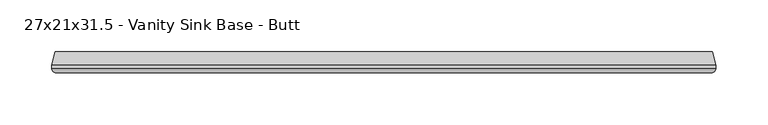
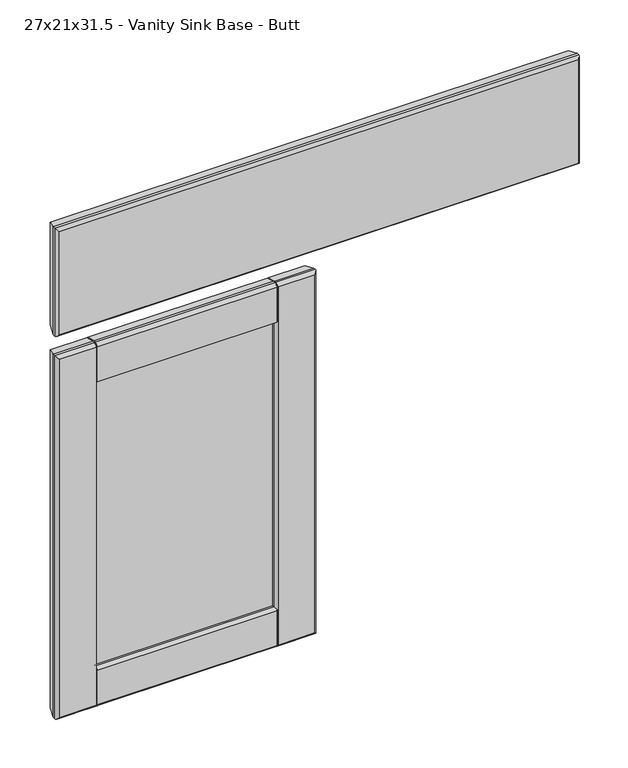
"""IFC4 building model written with IfcOpenShell, lengths in millimetres: furniture geometry, Cabinet-Base-Merillat-Double_Door-Marlin : 27x21x31.5 - Vanity Sink Base - Butt."""

from ifc_helpers import new_model, si_unit, frame, origin, place, context, project, spatial, polyline, circle_curve, ellipse_curve, outline, extrude, source, transform, mapped, element, save
from ifc_brep_helpers import plane_surface, cylinder_surface, advanced_brep


def furniture_27x21x31_5_vanity_sink_base_butt_8131d798(model_context):
    return source(origin(), model_context, "Body", "SolidModel", [
        advanced_brep(
        [(-298.8408026, -629.92, 771.6035075), (-298.8408026, -629.92, 638.0964925), (336.3162124, -629.92, 638.0964925), (336.3162124, -629.92, 771.6035075), (-298.4320951, -609.6, 638.5052), (-298.4320951, -609.6, 771.1948), (335.9075049, -609.6, 771.1948), (335.9075049, -609.6, 638.5052), (-301.9372951, -625.4496, 774.7), (-301.9372951, -622.681, 774.7), (-301.9372951, -622.681, 635.0), (-301.9372951, -625.4496, 635.0), (339.4127049, -622.681, 635.0), (339.4127049, -625.4496, 635.0), (339.4127049, -622.681, 774.7), (339.4127049, -625.4496, 774.7)],
        [
            (0, 1),
            (1, 2),
            (2, 3),
            (3, 0),
            (4, 5),
            (5, 6),
            (6, 7),
            (7, 4),
            (8, 9),
            (9, 10),
            (10, 11),
            (11, 8),
            (10, 12),
            (12, 13),
            (13, 11),
            (12, 14),
            (14, 15),
            (15, 13),
            (8, 15),
            (14, 9),
            (11, 1, ellipse_curve(frame((-297.1620951, -625.4496, 639.7752), z_axis=(-0.7071067811865475, 0.0, 0.7071067811865475), x_axis=(-0.7071067811865474, 0.0, -0.7071067811865476)), 6.7531526, 4.7752)),
            (0, 8, ellipse_curve(frame((-297.1620951, -625.4496, 769.9248), z_axis=(-0.7071067811865475, 0.0, -0.7071067811865475), x_axis=(0.7071067811865474, 0.0, -0.7071067811865476)), 6.7531526, 4.7752)),
            (4, 10),
            (9, 5),
            (13, 2, ellipse_curve(frame((334.6375049, -625.4496, 639.7752), z_axis=(-0.7071067811865475, 0.0, -0.7071067811865475), x_axis=(0.7071067811865476, 0.0, -0.7071067811865474)), 6.7531526, 4.7752)),
            (7, 12),
            (15, 3, ellipse_curve(frame((334.6375049, -625.4496, 769.9248), z_axis=(0.7071067811865475, 0.0, -0.7071067811865475), x_axis=(0.7071067811865474, 0.0, 0.7071067811865476)), 6.7531526, 4.7752)),
            (6, 14),
        ],
        [
            plane_surface(frame((-301.9372951, -629.92, 774.7), z_axis=(0.0, -1.0, 0.0), x_axis=(0.0, 0.0, -1.0))),
            plane_surface(frame((-301.9372951, -609.6, 774.7), z_axis=(0.0, 1.0, 0.0), x_axis=(0.0, 0.0, 1.0))),
            plane_surface(frame((-301.9372951, -629.92, 774.7), z_axis=(-1.0, 0.0, 0.0), x_axis=(0.0, 1.0, 0.0))),
            plane_surface(frame((-301.9372951, -629.92, 635.0), z_axis=(0.0, 0.0, -1.0), x_axis=(0.0, 1.0, 0.0))),
            plane_surface(frame((339.4127049, -629.92, 635.0), z_axis=(1.0, 0.0, 0.0), x_axis=(0.0, 1.0, 0.0))),
            plane_surface(frame((339.4127049, -629.92, 774.7), z_axis=(0.0, 0.0, 1.0), x_axis=(0.0, 1.0, 0.0))),
            cylinder_surface(frame((-297.1620951, -625.4496, 774.7), z_axis=(0.0, 0.0, -1.0), x_axis=(0.0, 1.0, 0.0)), 4.7752),
            plane_surface(frame((-301.9372951, -622.681, 774.7), z_axis=(-0.9659229350723619, 0.25882983502910506, 0.0), x_axis=(0.0, 0.0, -1.0))),
            cylinder_surface(frame((-301.9372951, -625.4496, 639.7752), z_axis=(1.0, 0.0, 0.0), x_axis=(0.0, 1.0, 0.0)), 4.7752),
            plane_surface(frame((-301.9372951, -622.681, 635.0), z_axis=(0.0, 0.25882983502910506, -0.9659229350723619), x_axis=(1.0, 0.0, 0.0))),
            cylinder_surface(frame((334.6375049, -625.4496, 635.0), z_axis=(0.0, 0.0, 1.0), x_axis=(0.0, 1.0, 0.0)), 4.7752),
            plane_surface(frame((339.4127049, -622.681, 635.0), z_axis=(0.9659229350723619, 0.25882983502910506, 0.0), x_axis=(0.0, 0.0, 1.0))),
            cylinder_surface(frame((339.4127049, -625.4496, 769.9248), z_axis=(-1.0, 0.0, 0.0), x_axis=(0.0, 1.0, 0.0)), 4.7752),
            plane_surface(frame((339.4127049, -622.681, 774.7), z_axis=(0.0, 0.25882983502910506, 0.9659229350723619), x_axis=(-1.0, 0.0, 0.0))),
        ],
        [
            (0, [[1, 2, 3, 4]]),
            (1, [[5, 6, 7, 8]]),
            (2, [[9, 10, 11, 12]]),
            (3, [[-11, 13, 14, 15]]),
            (4, [[-14, 16, 17, 18]]),
            (5, [[-9, 19, -17, 20]]),
            (6, [[21, -1, 22, -12]]),
            (7, [[23, -10, 24, -5]]),
            (8, [[-21, -15, 25, -2]]),
            (9, [[-23, -8, 26, -13]]),
            (10, [[-25, -18, 27, -3]]),
            (11, [[-26, -7, 28, -16]]),
            (12, [[-22, -4, -27, -19]]),
            (13, [[-24, -20, -28, -6]]),
        ],
    ),
        advanced_brep(
        [(-301.9372951, -625.4496, 609.6), (-301.9372951, -625.4496, 139.7), (-298.8408026, -629.92, 142.7964925), (-298.8408026, -629.92, 606.5035075), (-301.9372951, -622.681, 609.6), (-301.9372951, -622.681, 139.7), (-298.4320951, -609.6, 606.0948), (-298.4320951, -609.6, 143.2052), (-253.7361323, -609.6, 561.3988372), (-253.3660006, -610.39375, 561.0287055), (-251.2848416, -614.85681, 558.9475465), (-251.2848416, -614.85681, 190.3524535), (-253.3660006, -610.39375, 188.2712945), (-253.7361323, -609.6, 187.9011628), (-252.684611, -617.0969093, 560.347316), (-252.684611, -617.0969093, 188.952684), (-267.0122951, -617.347, 574.675), (-267.0122951, -617.347, 174.625), (-267.0122951, -622.173, 574.675), (-267.0122951, -622.173, 174.625), (-252.684611, -622.4230907, 560.347316), (-252.684611, -622.4230907, 188.952684), (-251.2848416, -624.66319, 558.9475465), (-251.2848416, -624.66319, 190.3524535), (-253.3660006, -629.12625, 561.0287055), (-253.7332649, -629.9138508, 561.3959698), (-253.7361323, -629.92, 187.9011628), (-253.3660006, -629.12625, 188.2712945), (14.0537124, -629.92, 142.7964925), (-31.0140137, -629.92, 142.7964925), (-31.0140137, -625.4496, 139.7), (17.1502049, -625.4496, 139.7), (-253.7332649, -625.4496, 139.7), (-253.7332649, -629.92, 142.7964925), (-252.1457649, -625.4496, 139.7), (-32.6015137, -625.4496, 139.7), (-32.6015137, -629.92, 142.7964925), (-252.1457649, -629.92, 142.7964925), (-31.0140137, -622.681, 139.7), (17.1502049, -622.681, 139.7), (-253.7332649, -622.681, 139.7), (-252.1457649, -622.681, 139.7), (-32.6015137, -622.681, 139.7), (-31.0140137, -609.6, 143.2052), (13.6450049, -609.6, 143.2052), (-252.1457649, -609.6, 143.2052), (-32.6015137, -609.6, 143.2052), (-253.7332649, -609.6, 143.2052), (-33.5022486, -614.85681, 190.3524535), (-31.4210895, -610.39375, 188.2712945), (-32.6015137, -610.39375, 188.2712945), (-32.6015137, -609.6, 187.9011628), (-252.1457649, -609.6, 187.9011628), (-252.1457649, -610.39375, 188.2712945), (-32.1024791, -617.0969093, 188.952684), (-17.7747951, -617.347, 174.625), (-17.7747951, -622.173, 174.625), (-32.1024791, -622.4230907, 188.952684), (-33.5022486, -624.66319, 190.3524535), (-252.1457649, -629.12625, 188.2712945), (-252.1457649, -629.92, 187.9011628), (-32.6015137, -629.92, 187.9011628), (-32.6015137, -629.12625, 188.2712945), (-31.4210895, -629.12625, 188.2712945), (17.1502049, -625.4496, 609.6), (14.0537124, -629.92, 606.5035075), (17.1502049, -622.681, 609.6), (13.6450049, -609.6, 606.0948), (-31.0509578, -609.6, 187.9011628), (-33.5022486, -614.85681, 558.9475465), (-31.4210895, -610.39375, 561.0287055), (-31.0509578, -609.6, 561.3988372), (-32.1024791, -617.0969093, 560.347316), (-17.7747951, -617.347, 574.675), (-17.7747951, -622.173, 574.675), (-32.1024791, -622.4230907, 560.347316), (-33.5022486, -624.66319, 558.9475465), (-31.0509578, -629.92, 187.9011628), (-31.0509578, -629.92, 561.3988372), (-31.4210895, -629.12625, 561.0287055), (-253.7332649, -629.92, 606.5035075), (-253.7332649, -625.4496, 609.6), (-31.0140137, -625.4496, 609.6), (-31.0140137, -629.92, 606.5035075), (-32.6015137, -625.4496, 609.6), (-252.1457649, -625.4496, 609.6), (-252.1457649, -629.92, 606.5035075), (-32.6015137, -629.92, 606.5035075), (-253.7332649, -622.681, 609.6), (-31.0140137, -622.681, 609.6), (-32.6015137, -622.681, 609.6), (-252.1457649, -622.681, 609.6), (-253.7332649, -609.6, 606.0948), (-31.0140137, -609.6, 606.0948), (-32.6015137, -609.6, 606.0948), (-252.1457649, -609.6, 606.0948), (-32.6015137, -609.6, 561.3988372), (-252.1457649, -609.6, 561.3988372), (-252.1457649, -610.39375, 561.0287055), (-32.6015137, -610.39375, 561.0287055), (-32.6015137, -629.12625, 561.0287055), (-32.6015137, -629.92, 561.3988372), (-252.1457649, -629.92, 561.3988372), (-252.1457649, -629.12625, 561.0287055), (-32.6015137, -629.12625, 606.3526052), (-32.6015137, -625.4496, 608.80625), (-32.6015137, -622.7855037, 608.80625), (-32.6015137, -610.39375, 605.4857412), (-31.0140137, -610.39375, 561.0287055), (-31.0140137, -610.39375, 605.4857412), (-31.0140137, -622.7855037, 608.80625), (-31.0140137, -625.4496, 608.80625), (-31.0140137, -629.12625, 606.3526052), (-31.0140137, -629.12625, 561.0287055), (-253.7332649, -629.12625, 561.0287055), (-253.7332649, -629.12625, 606.3526052), (-253.7332649, -625.4496, 608.80625), (-253.7332649, -622.7855037, 608.80625), (-253.7332649, -610.39375, 605.4857412), (-253.7332649, -610.39375, 561.0287055), (-252.1457649, -610.39375, 605.4857412), (-252.1457649, -622.7855037, 608.80625), (-252.1457649, -625.4496, 608.80625), (-252.1457649, -629.12625, 606.3526052), (-253.7332649, -610.39375, 188.2712945), (-253.7332649, -610.39375, 143.8142588), (-253.7332649, -622.7855037, 140.49375), (-253.7332649, -625.4496, 140.49375), (-253.7332649, -629.12625, 142.9473948), (-253.7332649, -629.12625, 188.2712945), (-252.1457649, -629.12625, 142.9473948), (-252.1457649, -625.4496, 140.49375), (-252.1457649, -622.7855037, 140.49375), (-252.1457649, -610.39375, 143.8142588), (-32.6015137, -610.39375, 143.8142588), (-32.6015137, -622.7855037, 140.49375), (-32.6015137, -625.4496, 140.49375), (-32.6015137, -629.12625, 142.9473948), (-31.0140137, -629.12625, 188.2712945), (-31.0140137, -629.12625, 142.9473948), (-31.0140137, -625.4496, 140.49375), (-31.0140137, -622.7855037, 140.49375), (-31.0140137, -610.39375, 143.8142588), (-31.0140137, -610.39375, 188.2712945)],
        [
            (0, 1),
            (1, 2, ellipse_curve(frame((-297.1620951, -625.4496, 144.4752), z_axis=(-0.7071067811865475, 0.0, 0.7071067811865475), x_axis=(0.7071067811865474, 0.0, 0.7071067811865476)), 6.7531526, 4.7752)),
            (2, 3),
            (3, 0, ellipse_curve(frame((-297.1620951, -625.4496, 604.8248), z_axis=(-0.7071067811865475, 0.0, -0.7071067811865475), x_axis=(-0.7071067811865474, 0.0, 0.7071067811865476)), 6.7531526, 4.7752)),
            (0, 4),
            (4, 5),
            (5, 1),
            (4, 6),
            (6, 7),
            (7, 5),
            (8, 9),
            (9, 10),
            (10, 11),
            (11, 12),
            (12, 13),
            (13, 8),
            (10, 14, ellipse_curve(frame((-252.7120951, -615.5223492, 560.3748), z_axis=(-0.7071067811865475, 0.0, -0.7071067811865475), x_axis=(-0.7071067811865474, 0.0, 0.7071067811865476)), 2.2271035, 1.5748)),
            (14, 15),
            (15, 11, ellipse_curve(frame((-252.7120951, -615.5223492, 188.9252), z_axis=(-0.7071067811865475, 0.0, 0.7071067811865475), x_axis=(0.7071067811865474, 0.0, 0.7071067811865476)), 2.2271035, 1.5748)),
            (14, 16),
            (16, 17),
            (17, 15),
            (16, 18),
            (18, 19),
            (19, 17),
            (18, 20),
            (20, 21),
            (21, 19),
            (20, 22, ellipse_curve(frame((-252.7120951, -623.9976508, 560.3748), z_axis=(-0.7071067811865475, 0.0, -0.7071067811865475), x_axis=(-0.7071067811865474, 0.0, 0.7071067811865476)), 2.2271035, 1.5748)),
            (22, 23),
            (23, 21, ellipse_curve(frame((-252.7120951, -623.9976508, 188.9252), z_axis=(-0.7071067811865475, 0.0, 0.7071067811865475), x_axis=(0.7071067811865474, 0.0, 0.7071067811865476)), 2.2271035, 1.5748)),
            (22, 24),
            (24, 25),
            (25, 26),
            (26, 27),
            (27, 23),
            (28, 29),
            (29, 30, circle_curve(frame((-31.0140137, -625.4496, 144.4752), z_axis=(1.0, 0.0, 0.0), x_axis=(0.0, 1.0, 0.0)), 4.7752)),
            (30, 31),
            (31, 28, ellipse_curve(frame((12.3750049, -625.4496, 144.4752), z_axis=(-0.7071067811865475, 0.0, -0.7071067811865475), x_axis=(-0.7071067811865476, 0.0, 0.7071067811865474)), 6.7531526, 4.7752)),
            (1, 32),
            (32, 33, circle_curve(frame((-253.7332649, -625.4496, 144.4752), z_axis=(-1.0, 0.0, 0.0), x_axis=(0.0, 1.0, 0.0)), 4.7752)),
            (33, 2),
            (34, 35),
            (35, 36, circle_curve(frame((-32.6015137, -625.4496, 144.4752), z_axis=(-1.0, 0.0, 0.0), x_axis=(0.0, 1.0, 0.0)), 4.7752)),
            (36, 37),
            (37, 34, circle_curve(frame((-252.1457649, -625.4496, 144.4752), z_axis=(1.0, 0.0, 0.0), x_axis=(0.0, 1.0, 0.0)), 4.7752)),
            (30, 38),
            (38, 39),
            (39, 31),
            (5, 40),
            (40, 32),
            (41, 42),
            (42, 35),
            (34, 41),
            (38, 43),
            (43, 44),
            (44, 39),
            (45, 46),
            (46, 42),
            (41, 45),
            (7, 47),
            (47, 40),
            (48, 49),
            (49, 50),
            (50, 51),
            (51, 52),
            (52, 53),
            (53, 12),
            (11, 48),
            (15, 54),
            (54, 48, ellipse_curve(frame((-32.0749951, -615.5223492, 188.9252), z_axis=(-0.7071067811865475, 0.0, -0.7071067811865475), x_axis=(-0.7071067811865476, 0.0, 0.7071067811865474)), 2.2271035, 1.5748)),
            (17, 55),
            (55, 54),
            (19, 56),
            (56, 55),
            (21, 57),
            (57, 56),
            (23, 58),
            (58, 57, ellipse_curve(frame((-32.0749951, -623.9976508, 188.9252), z_axis=(-0.7071067811865475, 0.0, -0.7071067811865475), x_axis=(-0.7071067811865476, 0.0, 0.7071067811865474)), 2.2271035, 1.5748)),
            (27, 59),
            (59, 60),
            (60, 61),
            (61, 62),
            (62, 63),
            (63, 58),
            (31, 64),
            (64, 65, ellipse_curve(frame((12.3750049, -625.4496, 604.8248), z_axis=(0.7071067811865475, 0.0, -0.7071067811865475), x_axis=(-0.7071067811865474, 0.0, -0.7071067811865476)), 6.7531526, 4.7752)),
            (65, 28),
            (39, 66),
            (66, 64),
            (44, 67),
            (67, 66),
            (68, 49),
            (48, 69),
            (69, 70),
            (70, 71),
            (71, 68),
            (54, 72),
            (72, 69, ellipse_curve(frame((-32.0749951, -615.5223492, 560.3748), z_axis=(0.7071067811865475, 0.0, -0.7071067811865475), x_axis=(-0.7071067811865474, 0.0, -0.7071067811865476)), 2.2271035, 1.5748)),
            (55, 73),
            (73, 72),
            (56, 74),
            (74, 73),
            (57, 75),
            (75, 74),
            (58, 76),
            (76, 75, ellipse_curve(frame((-32.0749951, -623.9976508, 560.3748), z_axis=(0.7071067811865475, 0.0, -0.7071067811865475), x_axis=(-0.7071067811865474, 0.0, -0.7071067811865476)), 2.2271035, 1.5748)),
            (63, 77),
            (77, 78),
            (78, 79),
            (79, 76),
            (3, 80),
            (80, 81, circle_curve(frame((-253.7332649, -625.4496, 604.8248), z_axis=(-1.0, 0.0, 0.0), x_axis=(0.0, 1.0, 0.0)), 4.7752)),
            (81, 0),
            (64, 82),
            (82, 83, circle_curve(frame((-31.0140137, -625.4496, 604.8248), z_axis=(1.0, 0.0, 0.0), x_axis=(0.0, 1.0, 0.0)), 4.7752)),
            (83, 65),
            (84, 85),
            (85, 86, circle_curve(frame((-252.1457649, -625.4496, 604.8248), z_axis=(1.0, 0.0, 0.0), x_axis=(0.0, 1.0, 0.0)), 4.7752)),
            (86, 87),
            (87, 84, circle_curve(frame((-32.6015137, -625.4496, 604.8248), z_axis=(-1.0, 0.0, 0.0), x_axis=(0.0, 1.0, 0.0)), 4.7752)),
            (81, 88),
            (88, 4),
            (66, 89),
            (89, 82),
            (90, 91),
            (91, 85),
            (84, 90),
            (88, 92),
            (92, 6),
            (67, 93),
            (93, 89),
            (94, 95),
            (95, 91),
            (90, 94),
            (51, 46),
            (45, 52),
            (43, 68),
            (71, 93),
            (92, 8),
            (13, 47),
            (96, 97),
            (97, 95),
            (94, 96),
            (9, 98),
            (98, 97),
            (96, 99),
            (99, 70),
            (69, 10),
            (72, 14),
            (73, 16),
            (74, 18),
            (75, 20),
            (76, 22),
            (79, 100),
            (100, 101),
            (101, 102),
            (102, 103),
            (103, 24),
            (33, 26),
            (25, 80),
            (36, 61),
            (60, 37),
            (83, 78),
            (77, 29),
            (86, 102),
            (101, 87),
            (100, 104),
            (104, 105, circle_curve(frame((-32.6015137, -625.4496, 604.8248), z_axis=(-1.0, 0.0, 0.0), x_axis=(0.0, 0.0, 1.0)), 3.98145)),
            (105, 106),
            (106, 107),
            (107, 99),
            (71, 108),
            (108, 109),
            (109, 110),
            (110, 111),
            (111, 112, circle_curve(frame((-31.0140137, -625.4496, 604.8248), z_axis=(1.0, 0.0, 0.0), x_axis=(0.0, 0.0, 1.0)), 3.98145)),
            (112, 113),
            (113, 78),
            (113, 79),
            (112, 104),
            (111, 105),
            (110, 106),
            (109, 107),
            (108, 70),
            (25, 114),
            (114, 115),
            (115, 116, circle_curve(frame((-253.7332649, -625.4496, 604.8248), z_axis=(-1.0, 0.0, 0.0), x_axis=(0.0, 0.0, 1.0)), 3.98145)),
            (116, 117),
            (117, 118),
            (118, 119),
            (119, 8),
            (98, 120),
            (120, 121),
            (121, 122),
            (122, 123, circle_curve(frame((-252.1457649, -625.4496, 604.8248), z_axis=(1.0, 0.0, 0.0), x_axis=(0.0, 0.0, 1.0)), 3.98145)),
            (123, 103),
            (24, 114),
            (123, 115),
            (122, 116),
            (121, 117),
            (120, 118),
            (9, 119),
            (13, 124),
            (124, 125),
            (125, 126),
            (126, 127),
            (127, 128, circle_curve(frame((-253.7332649, -625.4496, 144.4752), z_axis=(-1.0, 0.0, 0.0), x_axis=(0.0, 0.0, 1.0)), 3.98145)),
            (128, 129),
            (129, 26),
            (59, 130),
            (130, 131, circle_curve(frame((-252.1457649, -625.4496, 144.4752), z_axis=(1.0, 0.0, 0.0), x_axis=(0.0, 0.0, 1.0)), 3.98145)),
            (131, 132),
            (132, 133),
            (133, 53),
            (12, 124),
            (133, 125),
            (132, 126),
            (131, 127),
            (130, 128),
            (27, 129),
            (50, 134),
            (134, 135),
            (135, 136),
            (136, 137, circle_curve(frame((-32.6015137, -625.4496, 144.4752), z_axis=(-1.0, 0.0, 0.0), x_axis=(0.0, 0.0, 1.0)), 3.98145)),
            (137, 62),
            (138, 139),
            (139, 140, circle_curve(frame((-31.0140137, -625.4496, 144.4752), z_axis=(1.0, 0.0, 0.0), x_axis=(0.0, 0.0, 1.0)), 3.98145)),
            (140, 141),
            (141, 142),
            (142, 143),
            (143, 68),
            (77, 138),
            (63, 138),
            (143, 49),
            (142, 134),
            (141, 135),
            (140, 136),
            (139, 137),
        ],
        [
            cylinder_surface(frame((-297.1620951, -625.4496, 609.6), z_axis=(0.0, 0.0, 1.0), x_axis=(0.0, 1.0, 0.0)), 4.7752),
            plane_surface(frame((-301.9372951, -625.4496, 609.6), z_axis=(-1.0, 0.0, 0.0), x_axis=(0.0, 0.0, -1.0))),
            plane_surface(frame((-301.9372951, -622.681, 609.6), z_axis=(-0.9659229350723619, 0.25882983502910506, 0.0), x_axis=(0.0, 0.0, -1.0))),
            plane_surface(frame((-253.7361323, -609.6, 561.3988372), z_axis=(0.9063077870366099, 0.4226182617407856, 0.0), x_axis=(0.0, 0.0, -1.0))),
            cylinder_surface(frame((-252.7120951, -615.5223492, 609.6), z_axis=(0.0, 0.0, 1.0000000000000002), x_axis=(0.01745240643729364, -0.9998476951563912, 0.0)), 1.5748),
            plane_surface(frame((-252.684611, -617.0969093, 560.347316), z_axis=(0.017452406437322144, -0.9998476951563906, 0.0), x_axis=(0.0, 0.0, -1.0))),
            plane_surface(frame((-267.0122951, -617.347, 574.675), z_axis=(1.0, 0.0, 0.0), x_axis=(0.0, 0.0, -1.0))),
            plane_surface(frame((-267.0122951, -622.173, 574.675), z_axis=(0.01745240643727848, 0.9998476951563914, 0.0), x_axis=(0.0, 0.0, -1.0))),
            cylinder_surface(frame((-252.7120951, -623.9976508, 609.6), z_axis=(0.0, 0.0, 1.0000000000000002), x_axis=(0.9063077870367326, -0.42261826174052236, 0.0)), 1.5748),
            plane_surface(frame((-251.2848416, -624.66319, 558.9475465), z_axis=(0.9063077870366333, -0.4226182617407352, 0.0), x_axis=(0.0, 0.0, -1.0))),
            cylinder_surface(frame((-301.9372951, -625.4496, 144.4752), z_axis=(-1.0, 0.0, 0.0), x_axis=(0.0, 1.0, 0.0)), 4.7752),
            plane_surface(frame((-301.9372951, -625.4496, 139.7), z_axis=(0.0, 0.0, -1.0), x_axis=(1.0, 0.0, 0.0))),
            plane_surface(frame((-301.9372951, -622.681, 139.7), z_axis=(0.0, 0.25882983502910506, -0.9659229350723619), x_axis=(1.0, 0.0, 0.0))),
            plane_surface(frame((-253.7361323, -609.6, 187.9011628), z_axis=(0.0, 0.4226182617407856, 0.9063077870366099), x_axis=(1.0, 0.0, 0.0))),
            cylinder_surface(frame((-301.9372951, -615.5223492, 188.9252), z_axis=(-1.0000000000000002, 0.0, 0.0), x_axis=(0.0, -0.9998476951563912, 0.01745240643729364)), 1.5748),
            plane_surface(frame((-252.684611, -617.0969093, 188.952684), z_axis=(0.0, -0.9998476951563906, 0.017452406437322144), x_axis=(1.0, 0.0, 0.0))),
            plane_surface(frame((-267.0122951, -617.347, 174.625), z_axis=(0.0, 0.0, 1.0), x_axis=(1.0, 0.0, 0.0))),
            plane_surface(frame((-267.0122951, -622.173, 174.625), z_axis=(0.0, 0.9998476951563914, 0.01745240643727848), x_axis=(1.0, 0.0, 0.0))),
            cylinder_surface(frame((-301.9372951, -623.9976508, 188.9252), z_axis=(-1.0000000000000002, 0.0, 0.0), x_axis=(0.0, -0.42261826174052236, 0.9063077870367326)), 1.5748),
            plane_surface(frame((-251.2848416, -624.66319, 190.3524535), z_axis=(0.0, -0.4226182617407352, 0.9063077870366333), x_axis=(1.0, 0.0, 0.0))),
            cylinder_surface(frame((12.3750049, -625.4496, 139.7), z_axis=(0.0, 0.0, -1.0), x_axis=(0.0, 1.0, 0.0)), 4.7752),
            plane_surface(frame((17.1502049, -625.4496, 139.7), z_axis=(1.0, 0.0, 0.0), x_axis=(0.0, 0.0, 1.0))),
            plane_surface(frame((17.1502049, -622.681, 139.7), z_axis=(0.9659229350723619, 0.25882983502910506, 0.0), x_axis=(0.0, 0.0, 1.0))),
            plane_surface(frame((-31.0509578, -609.6, 187.9011628), z_axis=(-0.9063077870366099, 0.4226182617407856, 0.0), x_axis=(0.0, 0.0, 1.0))),
            cylinder_surface(frame((-32.0749951, -615.5223492, 139.7), z_axis=(0.0, 0.0, -1.0000000000000002), x_axis=(-0.01745240643729364, -0.9998476951563912, 0.0)), 1.5748),
            plane_surface(frame((-32.1024791, -617.0969093, 188.952684), z_axis=(-0.017452406437322144, -0.9998476951563906, 0.0), x_axis=(0.0, 0.0, 1.0))),
            plane_surface(frame((-17.7747951, -617.347, 174.625), z_axis=(-1.0, 0.0, 0.0), x_axis=(0.0, 0.0, 1.0))),
            plane_surface(frame((-17.7747951, -622.173, 174.625), z_axis=(-0.01745240643727848, 0.9998476951563914, 0.0), x_axis=(0.0, 0.0, 1.0))),
            cylinder_surface(frame((-32.0749951, -623.9976508, 139.7), z_axis=(0.0, 0.0, -1.0000000000000002), x_axis=(-0.9063077870367326, -0.42261826174052236, 0.0)), 1.5748),
            plane_surface(frame((-33.5022486, -624.66319, 190.3524535), z_axis=(-0.9063077870366333, -0.4226182617407352, 0.0), x_axis=(0.0, 0.0, 1.0))),
            cylinder_surface(frame((17.1502049, -625.4496, 604.8248), z_axis=(1.0, 0.0, 0.0), x_axis=(0.0, 1.0, 0.0)), 4.7752),
            plane_surface(frame((17.1502049, -625.4496, 609.6), z_axis=(0.0, 0.0, 1.0), x_axis=(-1.0, 0.0, 0.0))),
            plane_surface(frame((17.1502049, -622.681, 609.6), z_axis=(0.0, 0.25882983502910506, 0.9659229350723619), x_axis=(-1.0, 0.0, 0.0))),
            plane_surface(frame((13.6450049, -609.6, 606.0948), z_axis=(0.0, 1.0, 0.0), x_axis=(-1.0, 0.0, 0.0))),
            plane_surface(frame((-31.0509578, -609.6, 561.3988372), z_axis=(0.0, 0.4226182617407856, -0.9063077870366099), x_axis=(-1.0, 0.0, 0.0))),
            cylinder_surface(frame((17.1502049, -615.5223492, 560.3748), z_axis=(1.0000000000000002, 0.0, 0.0), x_axis=(0.0, -0.9998476951563912, -0.01745240643729364)), 1.5748),
            plane_surface(frame((-32.1024791, -617.0969093, 560.347316), z_axis=(0.0, -0.9998476951563906, -0.017452406437322144), x_axis=(-1.0, 0.0, 0.0))),
            plane_surface(frame((-17.7747951, -617.347, 574.675), z_axis=(0.0, 0.0, -1.0), x_axis=(-1.0, 0.0, 0.0))),
            plane_surface(frame((-17.7747951, -622.173, 574.675), z_axis=(0.0, 0.9998476951563914, -0.01745240643727848), x_axis=(-1.0, 0.0, 0.0))),
            cylinder_surface(frame((17.1502049, -623.9976508, 560.3748), z_axis=(1.0000000000000002, 0.0, 0.0), x_axis=(0.0, -0.42261826174052236, -0.9063077870367326)), 1.5748),
            plane_surface(frame((-33.5022486, -624.66319, 558.9475465), z_axis=(0.0, -0.4226182617407352, -0.9063077870366333), x_axis=(-1.0, 0.0, 0.0))),
            plane_surface(frame((-31.0509578, -629.92, 561.3988372), z_axis=(0.0, -1.0, 0.0), x_axis=(-1.0, 0.0, 0.0))),
            plane_surface(frame((-32.6015137, -629.92, 561.3988372), z_axis=(1.0, 0.0, 0.0), x_axis=(0.0, 0.9063077870366341, -0.4226182617407336))),
            plane_surface(frame((-31.0140137, -629.92, 561.3988372), z_axis=(-1.0, 0.0, 0.0), x_axis=(0.0, -0.9063077870366341, 0.4226182617407336))),
            plane_surface(frame((-32.6015137, -629.92, 561.3988372), z_axis=(0.0, 0.4226182617407336, 0.9063077870366341), x_axis=(1.0, 0.0, 0.0))),
            plane_surface(frame((-32.6015137, -629.12625, 561.0287055), z_axis=(0.0, -1.0, 0.0), x_axis=(1.0, 0.0, 0.0))),
            cylinder_surface(frame((-31.0140137, -625.4496, 604.8248), z_axis=(1.0, 0.0, 0.0), x_axis=(0.0, 0.0, 1.0)), 3.98145),
            plane_surface(frame((-32.6015137, -625.4496, 608.80625), z_axis=(0.0, 0.0, 1.0), x_axis=(1.0, 0.0, 0.0))),
            plane_surface(frame((-32.6015137, -622.7855037, 608.80625), z_axis=(0.0, 0.2588298350291669, 0.9659229350723454), x_axis=(1.0, 0.0, 0.0))),
            plane_surface(frame((-32.6015137, -610.39375, 605.4857412), z_axis=(0.0, 1.0, 0.0), x_axis=(1.0, 0.0, 0.0))),
            plane_surface(frame((-32.6015137, -610.39375, 561.0287055), z_axis=(0.0, -0.42261826174081096, 0.906307787036598), x_axis=(1.0, 0.0, 0.0))),
            plane_surface(frame((-253.7332649, -629.92, 561.3988372), z_axis=(1.0000000000000002, 0.0, 0.0), x_axis=(0.0, 0.9063077870366427, -0.42261826174071515))),
            plane_surface(frame((-252.1457649, -629.92, 561.3988372), z_axis=(-1.0000000000000002, 0.0, 0.0), x_axis=(0.0, -0.9063077870366427, 0.42261826174071515))),
            plane_surface(frame((-253.7332649, -629.92, 561.3988372), z_axis=(0.0, 0.42261826174071515, 0.9063077870366427), x_axis=(1.0, 0.0, 0.0))),
            plane_surface(frame((-253.7332649, -629.12625, 561.0287055), z_axis=(0.0, -1.0, 0.0), x_axis=(1.0, 0.0, 0.0))),
            cylinder_surface(frame((-252.1457649, -625.4496, 604.8248), z_axis=(1.0, 0.0, 0.0), x_axis=(0.0, 0.0, 1.0)), 3.98145),
            plane_surface(frame((-253.7332649, -625.4496, 608.80625), z_axis=(0.0, 0.0, 1.0), x_axis=(1.0, 0.0, 0.0))),
            plane_surface(frame((-253.7332649, -622.7855037, 608.80625), z_axis=(0.0, 0.25882983502916707, 0.9659229350723454), x_axis=(1.0, 0.0, 0.0))),
            plane_surface(frame((-253.7332649, -610.39375, 605.4857412), z_axis=(0.0, 1.0, 0.0), x_axis=(1.0, 0.0, 0.0))),
            plane_surface(frame((-253.7332649, -610.39375, 561.0287055), z_axis=(0.0, -0.42261826174082806, 0.9063077870365901), x_axis=(1.0, 0.0, 0.0))),
            plane_surface(frame((-253.7332649, -625.4496, 149.2504), z_axis=(1.0, 0.0, 0.0), x_axis=(0.0, -1.0, 0.0))),
            plane_surface(frame((-252.1457649, -625.4496, 149.2504), z_axis=(-1.0, 0.0, 0.0), x_axis=(0.0, 1.0, 0.0))),
            plane_surface(frame((-253.7332649, -609.6, 187.9011628), z_axis=(0.0, -0.4226182617407918, -0.906307787036607), x_axis=(1.0, 0.0, 0.0))),
            plane_surface(frame((-253.7332649, -610.39375, 188.2712945), z_axis=(0.0, 1.0, 0.0), x_axis=(1.0, 0.0, 0.0))),
            plane_surface(frame((-253.7332649, -610.39375, 143.8142588), z_axis=(0.0, 0.25882983502943513, -0.9659229350722734), x_axis=(1.0, 0.0, 0.0))),
            plane_surface(frame((-253.7332649, -622.7855037, 140.49375), z_axis=(0.0, 0.0, -1.0), x_axis=(1.0, 0.0, 0.0))),
            cylinder_surface(frame((-252.1457649, -625.4496, 144.4752), z_axis=(1.0, 0.0, 0.0), x_axis=(0.0, 0.0, 1.0)), 3.98145),
            plane_surface(frame((-253.7332649, -629.12625, 142.9473948), z_axis=(0.0, -1.0, 0.0), x_axis=(1.0, 0.0, 0.0))),
            plane_surface(frame((-253.7332649, -629.12625, 188.2712945), z_axis=(0.0, 0.42261826174073647, -0.9063077870366327), x_axis=(1.0, 0.0, 0.0))),
            plane_surface(frame((-32.6015137, -629.12625, 188.2712945), z_axis=(1.0, 0.0, 0.0), x_axis=(0.0, -0.9063077870366302, -0.42261826174074196))),
            plane_surface(frame((-31.0140137, -629.12625, 188.2712945), z_axis=(-1.0, 0.0, 0.0), x_axis=(0.0, 0.9063077870366302, 0.42261826174074196))),
            plane_surface(frame((-32.6015137, -629.12625, 188.2712945), z_axis=(0.0, 0.42261826174074196, -0.9063077870366302), x_axis=(1.0, 0.0, 0.0))),
            plane_surface(frame((-32.6015137, -609.6, 187.9011628), z_axis=(0.0, -0.4226182617408051, -0.9063077870366008), x_axis=(1.0, 0.0, 0.0))),
            plane_surface(frame((-32.6015137, -610.39375, 188.2712945), z_axis=(0.0, 1.0, 0.0), x_axis=(1.0, 0.0, 0.0))),
            plane_surface(frame((-32.6015137, -610.39375, 143.8142588), z_axis=(0.0, 0.258829835029436, -0.9659229350722733), x_axis=(1.0, 0.0, 0.0))),
            plane_surface(frame((-32.6015137, -622.7855037, 140.49375), z_axis=(0.0, 0.0, -1.0), x_axis=(1.0, 0.0, 0.0))),
            cylinder_surface(frame((-31.0140137, -625.4496, 144.4752), z_axis=(1.0, 0.0, 0.0), x_axis=(0.0, 0.0, 1.0)), 3.98145),
            plane_surface(frame((-32.6015137, -629.12625, 142.9473948), z_axis=(0.0, -1.0, 0.0), x_axis=(1.0, 0.0, 0.0))),
        ],
        [
            (0, [[1, 2, 3, 4]]),
            (1, [[5, 6, 7, -1]]),
            (2, [[8, 9, 10, -6]]),
            (3, [[11, 12, 13, 14, 15, 16]]),
            (4, [[17, 18, 19, -13]]),
            (5, [[20, 21, 22, -18]]),
            (6, [[23, 24, 25, -21]]),
            (7, [[26, 27, 28, -24]]),
            (8, [[29, 30, 31, -27]]),
            (9, [[32, 33, 34, 35, 36, -30]]),
            (10, [[37, 38, 39, 40]]),
            (10, [[41, 42, 43, -2]]),
            (10, [[44, 45, 46, 47]]),
            (11, [[-39, 48, 49, 50]]),
            (11, [[51, 52, -41, -7]]),
            (11, [[53, 54, -44, 55]]),
            (12, [[-49, 56, 57, 58]]),
            (12, [[59, 60, -53, 61]]),
            (12, [[62, 63, -51, -10]]),
            (13, [[64, 65, 66, 67, 68, 69, -14, 70]]),
            (14, [[71, 72, -70, -19]]),
            (15, [[73, 74, -71, -22]]),
            (16, [[75, 76, -73, -25]]),
            (17, [[77, 78, -75, -28]]),
            (18, [[79, 80, -77, -31]]),
            (19, [[-36, 81, 82, 83, 84, 85, 86, -79]]),
            (20, [[87, 88, 89, -40]]),
            (21, [[90, 91, -87, -50]]),
            (22, [[92, 93, -90, -58]]),
            (23, [[94, -64, 95, 96, 97, 98]]),
            (24, [[99, 100, -95, -72]]),
            (25, [[101, 102, -99, -74]]),
            (26, [[103, 104, -101, -76]]),
            (27, [[105, 106, -103, -78]]),
            (28, [[107, 108, -105, -80]]),
            (29, [[-86, 109, 110, 111, 112, -107]]),
            (30, [[113, 114, 115, -4]]),
            (30, [[116, 117, 118, -88]]),
            (30, [[119, 120, 121, 122]]),
            (31, [[-115, 123, 124, -5]]),
            (31, [[125, 126, -116, -91]]),
            (31, [[127, 128, -119, 129]]),
            (32, [[-124, 130, 131, -8]]),
            (32, [[132, 133, -125, -93]]),
            (32, [[134, 135, -127, 136]]),
            (33, [[-67, 137, -59, 138]]),
            (33, [[-57, 139, -98, 140, -132, -92]]),
            (33, [[-131, 141, -16, 142, -62, -9]]),
            (33, [[143, 144, -134, 145]]),
            (34, [[-12, 146, 147, -143, 148, 149, -96, 150]]),
            (35, [[-150, -100, 151, -17]]),
            (36, [[-151, -102, 152, -20]]),
            (37, [[-152, -104, 153, -23]]),
            (38, [[-153, -106, 154, -26]]),
            (39, [[-154, -108, 155, -29]]),
            (40, [[-112, 156, 157, 158, 159, 160, -32, -155]]),
            (41, [[-43, 161, -34, 162, -113, -3]]),
            (41, [[-46, 163, -83, 164]]),
            (41, [[-118, 165, -110, 166, -37, -89]]),
            (41, [[-121, 167, -158, 168]]),
            (42, [[-148, -145, -136, -129, -122, -168, -157, 169, 170, 171, 172, 173]]),
            (43, [[-165, -117, -126, -133, -140, 174, 175, 176, 177, 178, 179, 180]]),
            (44, [[181, -111, -180]]),
            (45, [[-156, -181, -179, 182, -169]]),
            (46, [[-182, -178, 183, -170]]),
            (47, [[-183, -177, 184, -171]]),
            (48, [[-184, -176, 185, -172]]),
            (49, [[-185, -175, 186, -149, -173]]),
            (50, [[-97, -186, -174]]),
            (51, [[-141, -130, -123, -114, -162, 187, 188, 189, 190, 191, 192, 193]]),
            (52, [[-159, -167, -120, -128, -135, -144, -147, 194, 195, 196, 197, 198]]),
            (53, [[-33, 199, -187]]),
            (54, [[-199, -160, -198, 200, -188]]),
            (55, [[-200, -197, 201, -189]]),
            (56, [[-201, -196, 202, -190]]),
            (57, [[-202, -195, 203, -191]]),
            (58, [[-203, -194, -146, 204, -192]]),
            (59, [[-204, -11, -193]]),
            (60, [[-161, -42, -52, -63, -142, 205, 206, 207, 208, 209, 210, 211]]),
            (61, [[-68, -138, -61, -55, -47, -164, -82, 212, 213, 214, 215, 216]]),
            (62, [[-15, 217, -205]]),
            (63, [[-217, -69, -216, 218, -206]]),
            (64, [[-218, -215, 219, -207]]),
            (65, [[-219, -214, 220, -208]]),
            (66, [[-220, -213, 221, -209]]),
            (67, [[-221, -212, -81, 222, -210]]),
            (68, [[-222, -35, -211]]),
            (69, [[-84, -163, -45, -54, -60, -137, -66, 223, 224, 225, 226, 227]]),
            (70, [[228, 229, 230, 231, 232, 233, -139, -56, -48, -38, -166, 234]]),
            (71, [[-109, 235, -234]]),
            (72, [[236, -94, -233]]),
            (73, [[-65, -236, -232, 237, -223]]),
            (74, [[-237, -231, 238, -224]]),
            (75, [[-238, -230, 239, -225]]),
            (76, [[-239, -229, 240, -226]]),
            (77, [[-240, -228, -235, -85, -227]]),
        ],
    ),
        extrude(outline(polyline([(-17.7747951, -622.173), (-267.0122951, -622.173), (-267.0122951, -617.347), (-17.7747951, -617.347), (-17.7747951, -622.173)])), frame((0.0, 0.0, 174.625), z_axis=(0.0, 0.0, 1.0), x_axis=(1.0, 0.0, 0.0)), (0.0, 0.0, 1.0), 400.05),
    ])


if __name__ == "__main__":
    model = new_model("IFC4")
    model_context = context("Model", 3, world=origin())
    ifc_project = project(units=[si_unit("LENGTHUNIT", "METRE", prefix="MILLI")], contexts=[model_context])
    site = spatial("IfcSite", under=ifc_project)
    building = spatial("IfcBuilding", under=site)
    placement = place(None, origin())
    furniture_27x21x31_5_vanity_sink_base_butt_shape = furniture_27x21x31_5_vanity_sink_base_butt_8131d798(model_context)
    element("IfcFurniture", 1, ObjectType="Cabinet-Base-Merillat-Double_Door-Marlin : 27x21x31.5 - Vanity Sink Base - Butt", at=placement, inside=building, context=model_context, shape_type="MappedRepresentation", body=[
        mapped(furniture_27x21x31_5_vanity_sink_base_butt_shape, transform((0.0, 0.0, 0.0), x_axis=(1.0, 0.0, 0.0), y_axis=(0.0, 1.0, 0.0), z_axis=(0.0, 0.0, 1.0))),
    ])
    save(model, "model.ifc")

# Revit data of these elements
# Type "Cabinet-Base-Merillat-Double_Door-Marlin : 27x21x31.5 - Vanity Sink Base - Butt"
#   URL = "http://www.merillat.com"
#   Toe Kick Note = "Toe Kick Covering is not included. To be purchased Separately."
#   Product Line = "Express"
#   Product Page URL = "http://www.merillat.com//our-products/rooms/bathroom"
#   Product Group = "Vanity Cabinet"
#   Product Documentation Link = "http://merillatbusiness.com/customer-resources/product-line-resources/merillat-classic/"
#   Model = "VSB30B"
#   Manufacturer = "Merillat"
#   Finish = "Wood"
#   Description = "Vanity Sink Base Butt Door"
#   Construction Type = "Deep Sink Base"
#   Cabinet Construction Note = "No shelf, cabinets w/ a \"B\" suffix have BUTT doors without a center frame stile,  VSB39, VSB42. VSB3935 and VSB4235 have a double door with a frame center stile, All cabinets have one full-width drawer front except VSB42 and VSB4235 which have two drawer fronts"
#   Assembly Code = "C1030410"
#   Toe Kick Height = 0' - 4 1/2"
#   Toe Kick Depth = 0' - 2 25/32"
#   Top and Bottom Spacing = 0' - 1"
#   Side Spacing = 0' - 0 7/8"
#   Cabinet Shell = 0' - 0 3/8"
#   Door Spacing = 0' - 0 1/8"
#   Depth = 1' - 9"
#   Height = 2' - 7 1/2"
#   Width = 2' - 3"
#   Cabinet Drawer Width = 2' - 1 1/4"
#   Cabinet Drawer Height = 0' - 5 1/2"
#   Cabinet Drawer 2 Drawer Width = 1' - 0 9/16"
#   Cabinet Door Width = 1' - 0 9/16"
#   Cabinet Door Height = 1' - 6 1/2"
#   COBie.Type = no
#   Two Drawer = no
#   Elevation Swing Line = yes
#   Partial Overlay = yes
#   One Drawer = yes
#   Full Overlay = no
#   Butt Option = yes
#   Toe Kick Material = Wood - Merillat - Raw Particle Board
#   Door Drawer Material = Wood - Merillat - Pecan(1)
#   Cabinet Material = Wood - Merillat - Pecan(1)
#   Cabinet Drawer Style 2 Drawer = element 819256
#   Cabinet Drawer Style = element 819255
#   Cabinet Door Style = element 819254
# Element 1 (IfcFurniture, "Cabinet-Base-Merillat-Double_Door-Marlin : 27x21x31.5 - Vanity Sink Base - Butt")
#   Materials on its faces: "Wood - Merillat - Pecan(1)", "Wood - Merillat - Raw Particle Board"
# Materials
#   "Wood - Merillat - Raw Particle Board": class "Plastic", colour RGB 80 80 80, transparency 0, Description = "Plastic Laminate - Navy", Cost = 0
#   "Wood - Merillat - Pecan(1)": class "Wood", colour RGB 108 67 43, transparency 0, Cost = 0
